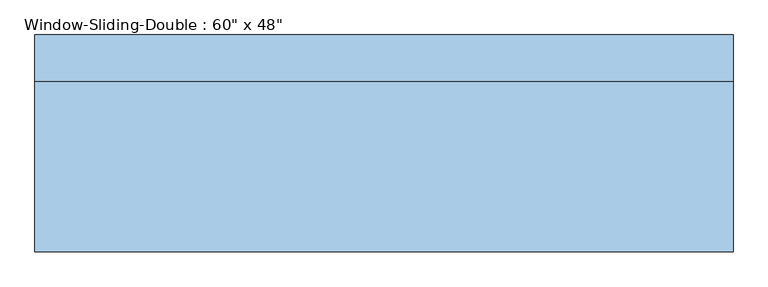
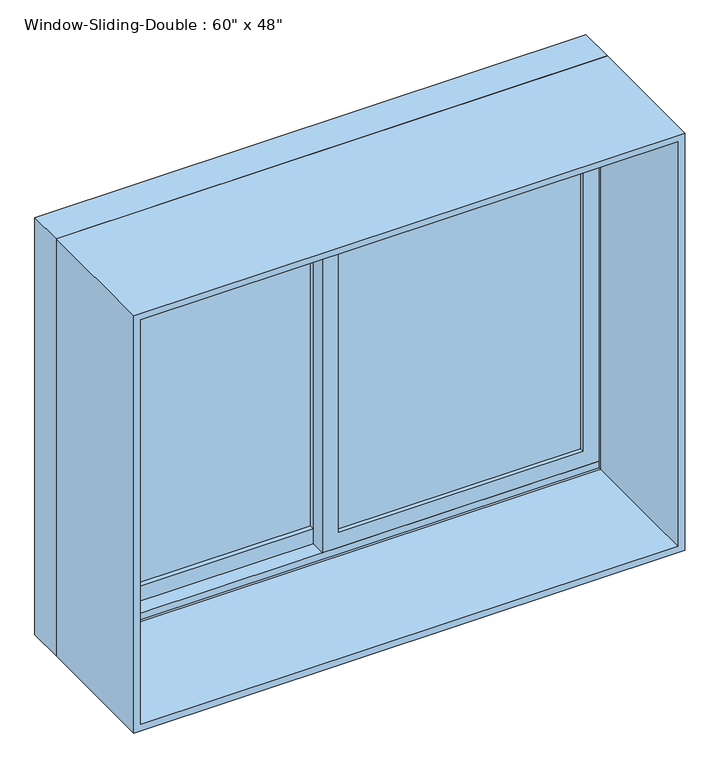
"""IFC4 building model written with IfcOpenShell, lengths in millimetres: window geometry."""

from ifc_helpers import new_model, si_unit, frame, origin, place, context, project, spatial, polyline, outline, extrude, faceted_brep, source, transform, mapped, element, save


def window_501efa1c(model_context):
    return source(origin(), model_context, "Body", "SolidModel", [
        faceted_brep([(-762.0, 140.6525, 914.4), (-762.0, 242.2525, 914.4), (762.0, 242.2525, 914.4), (762.0, 140.6525, 914.4), (-721.0778905, 242.2525, 2092.6778905), (-721.0778905, 235.9025, 2092.6778905), (-721.0778905, 235.9025, 933.45), (-721.0778905, 242.2525, 933.45), (721.0778905, 235.9025, 2092.6778905), (721.0778905, 235.9025, 933.45), (742.95, 235.9025, 933.45), (742.95, 235.9025, 2114.55), (-742.95, 235.9025, 2114.55), (-742.95, 235.9025, 933.45), (-742.95, 140.6525, 2114.55), (-742.95, 140.6525, 933.45), (-742.95, 147.0025, 933.45), (-742.95, 147.0025, 952.5), (-742.95, 191.4525, 952.5), (-742.95, 191.4525, 933.45), (762.0, 140.6525, 2133.6), (-762.0, 140.6525, 2133.6), (742.95, 140.6525, 2114.55), (742.95, 140.6525, 933.45), (-762.0, 242.2525, 2133.6), (762.0, 242.2525, 2133.6), (721.0778905, 242.2525, 933.45), (721.0778905, 242.2525, 2092.6778905), (742.95, 191.4525, 933.45), (742.95, 191.4525, 952.5), (742.95, 147.0025, 952.5), (742.95, 147.0025, 933.45)], [[[0, 1, 2, 3]], [[4, 5, 6, 7]], [[5, 8, 9, 10, 11, 12, 13, 6]], [[12, 14, 15, 16, 17, 18, 19, 13]], [[0, 3, 20, 21], [22, 23, 15, 14]], [[24, 1, 0, 21]], [[2, 1, 24, 25], [4, 7, 26, 27]], [[5, 4, 27, 8]], [[12, 11, 22, 14]], [[21, 20, 25, 24]], [[8, 27, 26, 9]], [[22, 11, 10, 28, 29, 30, 31, 23]], [[20, 3, 2, 25]], [[26, 7, 6, 13, 19, 28, 10, 9]], [[28, 19, 18, 29]], [[29, 18, 17, 30]], [[30, 17, 16, 31]], [[15, 23, 31, 16]]]),
        extrude(outline(polyline([(2133.6, -762.0), (914.4, -762.0), (914.4, 762.0), (2133.6, 762.0), (2133.6, -762.0)]), holes=[polyline([(2114.55, 742.95), (933.45, 742.95), (933.45, -742.95), (2114.55, -742.95), (2114.55, 742.95)])]), frame((0.0, -230.8225, 0.0), z_axis=(0.0, 1.0, 0.0), x_axis=(0.0, 0.0, 1.0)), (0.0, 0.0, 1.0), 371.475),
        extrude(outline(polyline([(698.5, 178.7525), (698.5, 172.4025), (22.225, 172.4025), (22.225, 178.7525), (698.5, 178.7525)])), frame((0.0, 0.0, 996.95), z_axis=(0.0, 0.0, 1.0), x_axis=(1.0, 0.0, 0.0)), (0.0, 0.0, 1.0), 1073.15),
        extrude(outline(polyline([(698.5, 166.0525), (698.5, 159.7025), (22.225, 159.7025), (22.225, 166.0525), (698.5, 166.0525)])), frame((0.0, 0.0, 996.95), z_axis=(0.0, 0.0, 1.0), x_axis=(1.0, 0.0, 0.0)), (0.0, 0.0, 1.0), 1073.15),
        extrude(outline(polyline([(-22.225, 223.2025), (-22.225, 216.8525), (-698.5, 216.8525), (-698.5, 223.2025), (-22.225, 223.2025)])), frame((0.0, 0.0, 996.95), z_axis=(0.0, 0.0, 1.0), x_axis=(1.0, 0.0, 0.0)), (0.0, 0.0, 1.0), 1073.15),
        extrude(outline(polyline([(-22.225, 210.5025), (-22.225, 204.1525), (-698.5, 204.1525), (-698.5, 210.5025), (-22.225, 210.5025)])), frame((0.0, 0.0, 996.95), z_axis=(0.0, 0.0, 1.0), x_axis=(1.0, 0.0, 0.0)), (0.0, 0.0, 1.0), 1073.15),
        extrude(outline(polyline([(933.45, -742.95), (933.45, 22.225), (2114.55, 22.225), (2114.55, -742.95), (933.45, -742.95)]), holes=[polyline([(2070.1, -22.225), (996.95, -22.225), (996.95, -698.5), (2070.1, -698.5), (2070.1, -22.225)])]), frame((0.0, 191.4525, 0.0), z_axis=(0.0, 1.0, 0.0), x_axis=(0.0, 0.0, 1.0)), (0.0, 0.0, 1.0), 44.45),
        extrude(outline(polyline([(952.5, 742.95), (2114.55, 742.95), (2114.55, -22.225), (952.5, -22.225), (952.5, 742.95)]), holes=[polyline([(996.95, 22.225), (2070.1, 22.225), (2070.1, 698.5), (996.95, 698.5), (996.95, 22.225)])]), frame((0.0, 147.0025, 0.0), z_axis=(0.0, 1.0, 0.0), x_axis=(0.0, 0.0, 1.0)), (0.0, 0.0, 1.0), 44.45),
    ])


if __name__ == "__main__":
    model = new_model("IFC4")
    model_context = context("Model", 3, world=origin())
    ifc_project = project(units=[si_unit("LENGTHUNIT", "METRE", prefix="MILLI")], contexts=[model_context])
    site = spatial("IfcSite", under=ifc_project)
    building = spatial("IfcBuilding", under=site)
    placement = place(None, origin())
    window_shape = window_501efa1c(model_context)
    element("IfcWindow", 1, ObjectType="Window-Sliding-Double : 60\" x 48\"", at=placement, inside=building, context=model_context, shape_type="MappedRepresentation", body=[
        mapped(window_shape, transform((0.0, 0.0, 0.0), x_axis=(1.0, 0.0, 0.0), y_axis=(0.0, 1.0, 0.0), z_axis=(0.0, 0.0, 1.0))),
    ])
    save(model, "model.ifc")

# Revit data of these elements
# Type "Window-Sliding-Double : 60\" x 48\""
#   Type Mark = "13"
#   Fire Rating = "0.5h"
#   Assembly Code = "B2020100"
#   Analytic Construction = "Double glazing - domestic"
#   Window Inset [instance default] = 0' - 0"
#   Wall Thickness [instance default] = 0' - 6"
#   Visual Light Transmittance = 0.81
#   Thermal Resistance (R) = 1.8146 (h·ft²·°F)/BTU
#   Solar Heat Gain Coefficient = 0.76
#   Muntin Width = 2' - 2 5/8"
#   Muntin Height = 3' - 6 1/4"
#   Interior Wall Closure [instance default] = 0' - 2 3/4"
#   Heat Transfer Coefficient (U) = 0.5511 BTU/(h·ft²·°F)
#   Frame Extension [instance default] = 0' - 0 1/4"
#   Exterior Wall Closure [instance default] = 0' - 1 1/4"
#   Rough Width = 5' - 0 1/2"
#   Rough Height = 4' - 0 1/2"
#   Height = 4' - 0"
#   Extension Jamb [instance default] = 0' - 2 3/4"
#   Default Sill Height = 3' - 0"
#   Width = 5' - 0"
#   Interior Trim Visibility [instance default] = yes
#   Indicator Visibility [instance default] = yes
#   Exterior Trim Visibility [instance default] = yes
#   Muntin Visibility = yes
#   Extension Jamb Visibility [instance default] = yes
#   Define Thermal Properties by = 1
#   Muntin Pattern = Muntin Pattern_2x2 : Muntin Pattern_2x2
#   Interior Trim Material = Cherry
#   Interior Trim = Trim-Window-Interior-Flat : Picture Frame
#   Interior Frame Material = Cherry
#   Glass Panel Material = Glass, Clear Glazing
#   Exterior Trim Material = PVC, Flexible
#   Exterior Trim = Trim-Window-Exterior-Flat : with Sill
#   Exterior Frame Material = PVC, Flexible
#   Wall Closure = (empty or 0)
# Element 1 (IfcWindow, "Window-Sliding-Double : 60\" x 48\"")
#   Wall Thickness = 1' - 5 7/8"
#   Extension Jamb = 1' - 2 5/8"
#   Materials on its faces: "Cherry", "Glass, Clear Glazing", "PVC, Flexible"
# Materials
#   "Cherry": class "Wood", colour RGB 157 77 38, transparency 0, Description = "Prunus Serotina", Cost = 0
#   "Glass, Clear Glazing": class "Glass", colour RGB 120 120 120, transparency 0, Description = "Clear glazing", Cost = 0
#   "PVC, Flexible": class "Plastic", colour RGB 178 178 178, transparency 0, Description = "Flexible polyvinyl chloride", Cost = 0
